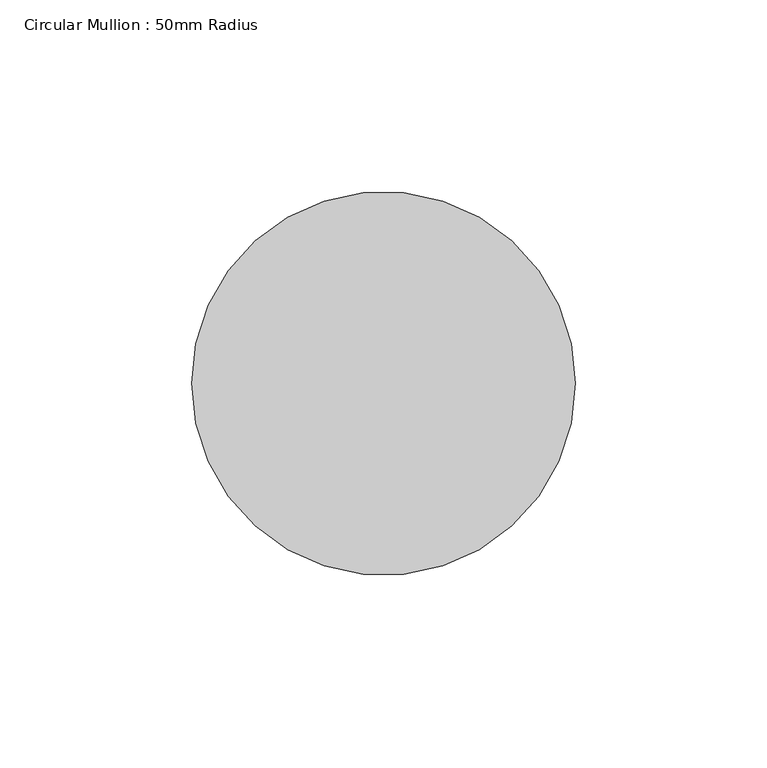
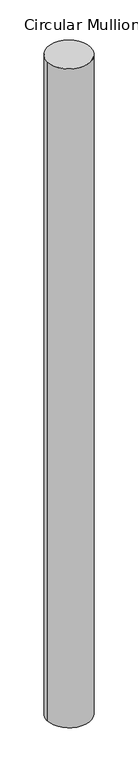
"""IFC4 building model written with IfcOpenShell, lengths in millimetres: member geometry, Circular Mullion : 50mm Radius."""

from ifc_helpers import new_model, si_unit, point, frame, origin, origin_2d, place, context, project, spatial, circle_curve, trimmed, segment, composite_curve, outline, extrude, source, transform, mapped, element, save


def circular_mullion_50mm_radius_6682cabd(model_context):
    return source(origin(), model_context, "Body", "SweptSolid", [
        extrude(outline(composite_curve([segment(trimmed(circle_curve(origin_2d(), 50.0), [point((50.0, 0.0))], [point((-50.0, 0.0))], False, "CARTESIAN"), True, "CONTINUOUS"), segment(trimmed(circle_curve(origin_2d(), 50.0), [point((-50.0, 0.0))], [point((50.0, 0.0))], False, "CARTESIAN"), True, "CONTINUOUS")], self_intersect=False)), frame((0.0, 0.0, -1602.0282222), z_axis=(0.0, 0.0, 1.0), x_axis=(1.0, 0.0, 0.0)), (0.0, 0.0, 1.0), 1602.0282222),
    ])


if __name__ == "__main__":
    model = new_model("IFC4")
    model_context = context("Model", 3, world=origin())
    ifc_project = project(units=[si_unit("LENGTHUNIT", "METRE", prefix="MILLI")], contexts=[model_context])
    site = spatial("IfcSite", under=ifc_project)
    building = spatial("IfcBuilding", under=site)
    placement = place(None, origin())
    circular_mullion_50mm_radius_shape = circular_mullion_50mm_radius_6682cabd(model_context)
    element("IfcMember", 1, ObjectType="Circular Mullion : 50mm Radius", at=placement, inside=building, context=model_context, shape_type="MappedRepresentation", body=[
        mapped(circular_mullion_50mm_radius_shape, transform((0.0, 0.0, 0.0), x_axis=(1.0, 0.0, 0.0), y_axis=(0.0, 1.0, 0.0), z_axis=(0.0, 0.0, 1.0))),
    ])
    save(model, "model.ifc")

# Revit data of these elements
# Type "Circular Mullion : 50mm Radius"
#   built-in parameter 1007350 = 0.164042 (stored number, unit not read)
# Element 1 (IfcMember, "Circular Mullion : 50mm Radius")
#   Materials on its faces: "Aluminium"
# Materials
#   "Aluminium": class "Metal", colour RGB 247 247 247, transparency 0, Description = "Aluminium 6061", Cost = 0
